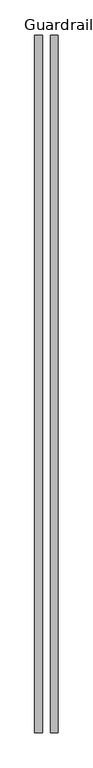
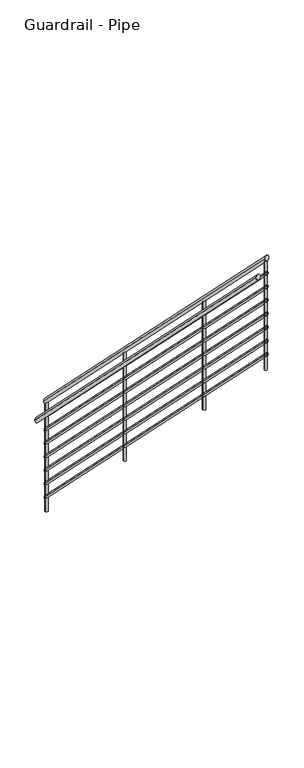
"""IFC4 building model written with IfcOpenShell, lengths in millimetres: railing geometry, Guardrail - Pipe."""

import ifcopenshell
import ifcopenshell.guid

model = None  # the IFC model being written
_history = None  # IfcOwnerHistory: only IFC2X3 demands one
_inside = {}  # id of a spatial element -> (the spatial element, [elements in it])
_under = {}  # id of a project, library or spatial element -> (it, [spatial elements below it])
_declared = {}  # id of a project -> (the project, [libraries it declares])
_typed = {}  # id of a type object -> (the type object, [elements of that type])
_made_of = {}  # id of a material, layer set ... -> (it, [elements and type objects made of it])


def new_model(schema):
    """Start an empty IFC model of exactly this schema.

    Asked for "IFC4X3", IfcOpenShell would pick the latest addendum, in which some entities
    have other attributes; the version numbers below select the first issue.
    IFC2X3 requires an IfcOwnerHistory on every rooted entity: one is made here for all.
    """
    global model, _history
    if schema == "IFC4X3":
        model = ifcopenshell.file(schema_version=(4, 3, 0, 0))
    else:
        model = ifcopenshell.file(schema=schema)
    _inside.clear()
    _under.clear()
    _declared.clear()
    _typed.clear()
    _made_of.clear()
    _history = None
    if model.schema == "IFC2X3":
        org = make("IfcOrganization", Name="unknown")
        user = make(
            "IfcPersonAndOrganization",
            ThePerson=make("IfcPerson", FamilyName="unknown"),
            TheOrganization=org,
        )
        app = make(
            "IfcApplication",
            ApplicationDeveloper=org,
            Version="unknown",
            ApplicationFullName="unknown",
            ApplicationIdentifier="unknown",
        )
        _history = make(
            "IfcOwnerHistory",
            OwningUser=user,
            OwningApplication=app,
            ChangeAction="ADDED",
            CreationDate=0,
        )
    return model


def make(cls, **values):
    """One entity of the class cls with the attributes given. An attribute that is None is left unset."""
    return model.create_entity(
        cls, **{name: value for name, value in values.items() if value is not None}
    )


def rooted(cls, **values):
    """An entity with a GlobalId (a new one), such as an element, a storey or a relation."""
    return make(cls, GlobalId=ifcopenshell.guid.new(), OwnerHistory=_history, **values)


def si_unit(unit_type, name, prefix=None):
    """IfcSIUnit, for example si_unit("LENGTHUNIT", "METRE", prefix="MILLI")."""
    return make("IfcSIUnit", UnitType=unit_type, Prefix=prefix, Name=name)


def assignment(units):
    """IfcUnitAssignment: the units of a project."""
    return None if units is None else make("IfcUnitAssignment", Units=units)


def point(xyz):
    """IfcCartesianPoint."""
    return None if xyz is None else make("IfcCartesianPoint", Coordinates=xyz)


def direction(xyz):
    """IfcDirection."""
    return None if xyz is None else make("IfcDirection", DirectionRatios=xyz)


def frame(location, z_axis=None, x_axis=None):
    """IfcAxis2Placement3D, a coordinate frame: its origin and axes. An axis left out is left unset."""
    return make(
        "IfcAxis2Placement3D",
        Location=point(location),
        Axis=direction(z_axis),
        RefDirection=direction(x_axis),
    )


def origin():
    """The frame at (0, 0, 0) with its axes left unset."""
    return frame((0.0, 0.0, 0.0))


def place(relative_to, where):
    """IfcLocalPlacement: puts the frame where relative to a parent placement (None: the world)."""
    return make(
        "IfcLocalPlacement", PlacementRelTo=relative_to, RelativePlacement=where
    )


def context(
    kind, dimensions, precision=None, world=None, true_north=None, identifier=None
):
    """IfcGeometricRepresentationContext, for example the 3D "Model" context."""
    return make(
        "IfcGeometricRepresentationContext",
        ContextIdentifier=identifier,
        ContextType=kind,
        CoordinateSpaceDimension=dimensions,
        Precision=precision,
        WorldCoordinateSystem=world,
        TrueNorth=true_north,
    )


def project(units=None, contexts=None):
    """IfcProject with its units and contexts."""
    return rooted(
        "IfcProject",
        Name="project",
        RepresentationContexts=contexts,
        UnitsInContext=assignment(units),
    )


def spatial(cls, under=None, at=None, **own):
    """A site, building, storey or space (cls), placed at a placement, below another one or the project."""
    s = rooted(cls, ObjectPlacement=at, **own)
    if under is not None:
        _under.setdefault(under.id(), (under, []))[1].append(s)
    return s


def circle_curve(where, radius):
    """IfcCircle in the frame where."""
    return make("IfcCircle", Position=where, Radius=radius)


def ellipse_curve(where, semi_axis1, semi_axis2):
    """IfcEllipse in the frame where."""
    return make(
        "IfcEllipse", Position=where, SemiAxis1=semi_axis1, SemiAxis2=semi_axis2
    )


def shape(context_of_items, identifier, shape_type, items):
    """IfcShapeRepresentation: the items that make up one representation, for example the "Body"."""
    return make(
        "IfcShapeRepresentation",
        ContextOfItems=context_of_items,
        RepresentationIdentifier=identifier,
        RepresentationType=shape_type,
        Items=items,
    )


def source(mapping_origin, context_of_items, identifier, shape_type, items):
    """IfcRepresentationMap: a shape defined once, which mapped items show again and again."""
    return make(
        "IfcRepresentationMap",
        MappingOrigin=mapping_origin,
        MappedRepresentation=shape(context_of_items, identifier, shape_type, items),
    )


def transform(
    local_origin,
    x_axis=None,
    y_axis=None,
    z_axis=None,
    scale=None,
    scale2=None,
    scale3=None,
    uniform=True,
):
    """IfcCartesianTransformationOperator3D, or its non-uniform kind. x_axis, y_axis, z_axis: its Axis1, 2, 3."""
    if uniform:
        return make(
            "IfcCartesianTransformationOperator3D",
            Axis1=direction(x_axis),
            Axis2=direction(y_axis),
            LocalOrigin=point(local_origin),
            Scale=scale,
            Axis3=direction(z_axis),
        )
    return make(
        "IfcCartesianTransformationOperator3DnonUniform",
        Axis1=direction(x_axis),
        Axis2=direction(y_axis),
        LocalOrigin=point(local_origin),
        Scale=scale,
        Axis3=direction(z_axis),
        Scale2=scale2,
        Scale3=scale3,
    )


def mapped(mapping_source, mapping_target):
    """IfcMappedItem: shows the shape of a source again, moved by a transform."""
    return make(
        "IfcMappedItem", MappingSource=mapping_source, MappingTarget=mapping_target
    )


def made_of(thing, what):
    """Note that an element or type object is made of a material, layer set ...; save() writes the relation."""
    if what is not None:
        _made_of.setdefault(what.id(), (what, []))[1].append(thing)
    return thing


def element(
    cls,
    number,
    at=None,
    inside=None,
    cuts=None,
    type_object=None,
    material=None,
    context=None,
    identifier="Body",
    shape_type=None,
    held_by="IfcProductDefinitionShape",
    body=None,
    shapes=None,
    **own,
):
    """One element of the class cls, such as IfcWall. Its Tag is "e" and its number.

    at: its placement. inside: the storey or other place that contains it. cuts: it is an
    opening in that element (IfcRelVoidsElement). A single representation is given by context,
    identifier, shape_type and body (its items); several are given by shapes. held_by: the class
    of the entity that holds the representations. save() writes the other relations.
    """
    e = rooted(cls, Tag="e%d" % number, ObjectPlacement=at, **own)
    if body is not None:
        shapes = [shape(context, identifier, shape_type, body)]
    if shapes is not None:
        e.Representation = make(held_by, Representations=shapes)
    if inside is not None:
        _inside.setdefault(inside.id(), (inside, []))[1].append(e)
    if cuts is not None:
        rooted(
            "IfcRelVoidsElement", RelatingBuildingElement=cuts, RelatedOpeningElement=e
        )
    if type_object is not None:
        _typed.setdefault(type_object.id(), (type_object, []))[1].append(e)
    return made_of(e, material)


def aggregate(whole, parts):
    """IfcRelAggregates: a whole, such as a stair, and the parts it consists of."""
    return rooted("IfcRelAggregates", RelatingObject=whole, RelatedObjects=parts)


def save(model, path):
    """Write the relations noted so far, then the file.

    IfcRelAggregates (storeys below a building ...), IfcRelContainedInSpatialStructure (elements
    in a storey), IfcRelDefinesByType, IfcRelAssociatesMaterial and IfcRelDeclares: one each for
    every whole, place, type object, material and project.
    """
    for whole, parts in _under.values():
        aggregate(whole, parts)
    for where, things in _inside.values():
        rooted(
            "IfcRelContainedInSpatialStructure",
            RelatedElements=things,
            RelatingStructure=where,
        )
    for kind, things in _typed.values():
        rooted("IfcRelDefinesByType", RelatedObjects=things, RelatingType=kind)
    for what, things in _made_of.values():
        rooted("IfcRelAssociatesMaterial", RelatedObjects=things, RelatingMaterial=what)
    for by, libraries in _declared.values():
        rooted("IfcRelDeclares", RelatingContext=by, RelatedDefinitions=libraries)
    model.write(path)


def plane_surface(at):
    """IfcPlane: the flat surface through the origin of the frame at, square to its z axis."""
    return make("IfcPlane", Position=at)


def cylinder_surface(at, radius):
    """IfcCylindricalSurface: all points at the distance radius from the z axis of the frame at."""
    return make("IfcCylindricalSurface", Position=at, Radius=radius)


def advanced_brep(points, edges, surfaces, faces):
    """IfcAdvancedBrep: a solid bounded by faces that lie on surfaces and meet in shared edges.

    An edge is (start, end): straight between two places in points (the first is 0);
    or (start, end, curve); or (start, end, curve, False) where it runs against its curve.
    A face is (place in surfaces, loops), or (place, loops, False) where it looks against
    its surface's normal. A loop lists edges by number (the first is 1), with a minus sign
    where the edge is run from its end to its start. The first loop is the outer one.
    """
    corners = [point(p) for p in points]
    vertices = [make("IfcVertexPoint", VertexGeometry=c) for c in corners]
    made = []
    for start, end, *more in edges:
        made.append(
            make(
                "IfcEdgeCurve",
                EdgeStart=vertices[start],
                EdgeEnd=vertices[end],
                EdgeGeometry=more[0] if more else make("IfcPolyline", Points=[corners[start], corners[end]]),
                SameSense=more[1] if len(more) > 1 else True,
            )
        )
    hull = []
    for where, loops, *sense in faces:
        bounds = []
        for j, loop in enumerate(loops):
            ring = [make("IfcOrientedEdge", EdgeElement=made[abs(k) - 1], Orientation=k > 0) for k in loop]
            bounds.append(
                make(
                    "IfcFaceOuterBound" if j == 0 else "IfcFaceBound",
                    Bound=make("IfcEdgeLoop", EdgeList=ring),
                    Orientation=True,
                )
            )
        hull.append(make("IfcAdvancedFace", Bounds=bounds, FaceSurface=surfaces[where], SameSense=sense[0] if sense else True))
    return make("IfcAdvancedBrep", Outer=make("IfcClosedShell", CfsFaces=hull))


def guardrail_pipe_ffde7d2e(model_context):
    return source(origin(), model_context, "Body", "AdvancedBrep", [
        advanced_brep(
        [(-590.6362718, 32344.1921646, 1268.4592316), (-552.5362718, 32344.1921646, 1268.4592316), (-590.6362718, 28942.3977925, 4670.2536037), (-552.5362718, 28942.3977925, 4670.2536037)],
        [
            (0, 1, ellipse_curve(frame((-571.5862718, 32344.1921646, 1268.4592316), z_axis=(0.0, 1.0, 0.0), x_axis=(0.0, 0.0, -1.0)), 26.9407684, 19.05)),
            (1, 0, ellipse_curve(frame((-571.5862718, 32344.1921646, 1268.4592316), z_axis=(0.0, 1.0, 0.0), x_axis=(0.0, 0.0, -1.0)), 26.9407684, 19.05)),
            (2, 3, ellipse_curve(frame((-571.5862718, 28942.3977925, 4670.2536037), z_axis=(0.0, -1.0, 0.0), x_axis=(0.0, 0.0, -1.0)), 26.9407684, 19.05)),
            (3, 2, ellipse_curve(frame((-571.5862718, 28942.3977925, 4670.2536037), z_axis=(0.0, -1.0, 0.0), x_axis=(0.0, 0.0, -1.0)), 26.9407684, 19.05)),
            (0, 2),
            (3, 1),
        ],
        [
            plane_surface(frame((-571.5862718, 32344.1921646, 1295.4), z_axis=(0.0, 1.0, 0.0), x_axis=(0.0, 0.0, -1.0))),
            plane_surface(frame((-571.5862718, 28942.3977925, 4697.194372), z_axis=(0.0, -1.0, 0.0), x_axis=(0.0, 0.0, -1.0))),
            cylinder_surface(frame((-571.5862718, 32330.7217804, 1281.9296158), z_axis=(0.0, 0.7071067811865476, -0.7071067811865476), x_axis=(1.0, 0.0, 0.0)), 19.05),
        ],
        [
            (0, [[1, 2]]),
            (1, [[3, 4]]),
            (2, [[-1, 5, -4, 6]]),
            (2, [[-2, -6, -3, -5]]),
        ],
    ),
        advanced_brep(
        [(-584.2862718, 32344.1921646, 1125.0394878), (-558.8862718, 32344.1921646, 1125.0394878), (-584.2862718, 28942.3977925, 4526.8338598), (-558.8862718, 28942.3977925, 4526.8338598)],
        [
            (0, 1, ellipse_curve(frame((-571.5862718, 32344.1921646, 1125.0394878), z_axis=(0.0, 1.0, 0.0), x_axis=(0.0, 0.0, -1.0)), 17.9605122, 12.7)),
            (1, 0, ellipse_curve(frame((-571.5862718, 32344.1921646, 1125.0394878), z_axis=(0.0, 1.0, 0.0), x_axis=(0.0, 0.0, -1.0)), 17.9605122, 12.7)),
            (2, 3, ellipse_curve(frame((-571.5862718, 28942.3977925, 4526.8338598), z_axis=(0.0, -1.0, 0.0), x_axis=(0.0, 0.0, -1.0)), 17.9605122, 12.7)),
            (3, 2, ellipse_curve(frame((-571.5862718, 28942.3977925, 4526.8338598), z_axis=(0.0, -1.0, 0.0), x_axis=(0.0, 0.0, -1.0)), 17.9605122, 12.7)),
            (0, 2),
            (3, 1),
        ],
        [
            plane_surface(frame((-571.5862718, 32344.1921646, 1143.0), z_axis=(0.0, 1.0, 0.0), x_axis=(0.0, 0.0, -1.0))),
            plane_surface(frame((-571.5862718, 28942.3977925, 4544.794372), z_axis=(0.0, -1.0, 0.0), x_axis=(0.0, 0.0, -1.0))),
            cylinder_surface(frame((-571.5862718, 32335.2119084, 1134.0197439), z_axis=(0.0, 0.7071067811865476, -0.7071067811865476), x_axis=(1.0, 0.0, 0.0)), 12.7),
        ],
        [
            (0, [[1, 2]]),
            (1, [[3, 4]]),
            (2, [[-1, 5, -4, 6]]),
            (2, [[-2, -6, -3, -5]]),
        ],
    ),
        advanced_brep(
        [(-666.8362718, 32344.1921646, 1116.0592316), (-628.7362718, 32344.1921646, 1116.0592316), (-666.8362718, 28942.3977925, 4517.8536037), (-628.7362718, 28942.3977925, 4517.8536037)],
        [
            (0, 1, ellipse_curve(frame((-647.7862718, 32344.1921646, 1116.0592316), z_axis=(0.0, 1.0, 0.0), x_axis=(0.0, 0.0, -1.0)), 26.9407684, 19.05)),
            (1, 0, ellipse_curve(frame((-647.7862718, 32344.1921646, 1116.0592316), z_axis=(0.0, 1.0, 0.0), x_axis=(0.0, 0.0, -1.0)), 26.9407684, 19.05)),
            (2, 3, ellipse_curve(frame((-647.7862718, 28942.3977925, 4517.8536037), z_axis=(0.0, -1.0, 0.0), x_axis=(0.0, 0.0, -1.0)), 26.9407684, 19.05)),
            (3, 2, ellipse_curve(frame((-647.7862718, 28942.3977925, 4517.8536037), z_axis=(0.0, -1.0, 0.0), x_axis=(0.0, 0.0, -1.0)), 26.9407684, 19.05)),
            (0, 2),
            (3, 1),
        ],
        [
            plane_surface(frame((-647.7862718, 32344.1921646, 1143.0), z_axis=(0.0, 1.0, 0.0), x_axis=(0.0, 0.0, -1.0))),
            plane_surface(frame((-647.7862718, 28942.3977925, 4544.794372), z_axis=(0.0, -1.0, 0.0), x_axis=(0.0, 0.0, -1.0))),
            cylinder_surface(frame((-647.7862718, 32330.7217804, 1129.5296158), z_axis=(0.0, 0.7071067811865476, -0.7071067811865476), x_axis=(1.0, 0.0, 0.0)), 19.05),
        ],
        [
            (0, [[1, 2]]),
            (1, [[3, 4]]),
            (2, [[-1, 5, -4, 6]]),
            (2, [[-2, -6, -3, -5]]),
        ],
    ),
        advanced_brep(
        [(-584.2862718, 32344.1921646, 998.0394878), (-558.8862718, 32344.1921646, 998.0394878), (-584.2862718, 28942.3977925, 4399.8338598), (-558.8862718, 28942.3977925, 4399.8338598)],
        [
            (0, 1, ellipse_curve(frame((-571.5862718, 32344.1921646, 998.0394878), z_axis=(0.0, 1.0, 0.0), x_axis=(0.0, 0.0, -1.0)), 17.9605122, 12.7)),
            (1, 0, ellipse_curve(frame((-571.5862718, 32344.1921646, 998.0394878), z_axis=(0.0, 1.0, 0.0), x_axis=(0.0, 0.0, -1.0)), 17.9605122, 12.7)),
            (2, 3, ellipse_curve(frame((-571.5862718, 28942.3977925, 4399.8338598), z_axis=(0.0, -1.0, 0.0), x_axis=(0.0, 0.0, -1.0)), 17.9605122, 12.7)),
            (3, 2, ellipse_curve(frame((-571.5862718, 28942.3977925, 4399.8338598), z_axis=(0.0, -1.0, 0.0), x_axis=(0.0, 0.0, -1.0)), 17.9605122, 12.7)),
            (0, 2),
            (3, 1),
        ],
        [
            plane_surface(frame((-571.5862718, 32344.1921646, 1016.0), z_axis=(0.0, 1.0, 0.0), x_axis=(0.0, 0.0, -1.0))),
            plane_surface(frame((-571.5862718, 28942.3977925, 4417.794372), z_axis=(0.0, -1.0, 0.0), x_axis=(0.0, 0.0, -1.0))),
            cylinder_surface(frame((-571.5862718, 32335.2119084, 1007.0197439), z_axis=(0.0, 0.7071067811865476, -0.7071067811865476), x_axis=(1.0, 0.0, 0.0)), 12.7),
        ],
        [
            (0, [[1, 2]]),
            (1, [[3, 4]]),
            (2, [[-1, 5, -4, 6]]),
            (2, [[-2, -6, -3, -5]]),
        ],
    ),
        advanced_brep(
        [(-584.2862718, 32344.1921646, 871.0394878), (-558.8862718, 32344.1921646, 871.0394878), (-584.2862718, 28942.3977925, 4272.8338598), (-558.8862718, 28942.3977925, 4272.8338598)],
        [
            (0, 1, ellipse_curve(frame((-571.5862718, 32344.1921646, 871.0394878), z_axis=(0.0, 1.0, 0.0), x_axis=(0.0, 0.0, -1.0)), 17.9605122, 12.7)),
            (1, 0, ellipse_curve(frame((-571.5862718, 32344.1921646, 871.0394878), z_axis=(0.0, 1.0, 0.0), x_axis=(0.0, 0.0, -1.0)), 17.9605122, 12.7)),
            (2, 3, ellipse_curve(frame((-571.5862718, 28942.3977925, 4272.8338598), z_axis=(0.0, -1.0, 0.0), x_axis=(0.0, 0.0, -1.0)), 17.9605122, 12.7)),
            (3, 2, ellipse_curve(frame((-571.5862718, 28942.3977925, 4272.8338598), z_axis=(0.0, -1.0, 0.0), x_axis=(0.0, 0.0, -1.0)), 17.9605122, 12.7)),
            (0, 2),
            (3, 1),
        ],
        [
            plane_surface(frame((-571.5862718, 32344.1921646, 889.0), z_axis=(0.0, 1.0, 0.0), x_axis=(0.0, 0.0, -1.0))),
            plane_surface(frame((-571.5862718, 28942.3977925, 4290.794372), z_axis=(0.0, -1.0, 0.0), x_axis=(0.0, 0.0, -1.0))),
            cylinder_surface(frame((-571.5862718, 32335.2119084, 880.0197439), z_axis=(0.0, 0.7071067811865476, -0.7071067811865476), x_axis=(1.0, 0.0, 0.0)), 12.7),
        ],
        [
            (0, [[1, 2]]),
            (1, [[3, 4]]),
            (2, [[-1, 5, -4, 6]]),
            (2, [[-2, -6, -3, -5]]),
        ],
    ),
        advanced_brep(
        [(-584.2862718, 32344.1921646, 744.0394878), (-558.8862718, 32344.1921646, 744.0394878), (-584.2862718, 28942.3977925, 4145.8338598), (-558.8862718, 28942.3977925, 4145.8338598)],
        [
            (0, 1, ellipse_curve(frame((-571.5862718, 32344.1921646, 744.0394878), z_axis=(0.0, 1.0, 0.0), x_axis=(0.0, 0.0, -1.0)), 17.9605122, 12.7)),
            (1, 0, ellipse_curve(frame((-571.5862718, 32344.1921646, 744.0394878), z_axis=(0.0, 1.0, 0.0), x_axis=(0.0, 0.0, -1.0)), 17.9605122, 12.7)),
            (2, 3, ellipse_curve(frame((-571.5862718, 28942.3977925, 4145.8338598), z_axis=(0.0, -1.0, 0.0), x_axis=(0.0, 0.0, -1.0)), 17.9605122, 12.7)),
            (3, 2, ellipse_curve(frame((-571.5862718, 28942.3977925, 4145.8338598), z_axis=(0.0, -1.0, 0.0), x_axis=(0.0, 0.0, -1.0)), 17.9605122, 12.7)),
            (0, 2),
            (3, 1),
        ],
        [
            plane_surface(frame((-571.5862718, 32344.1921646, 762.0), z_axis=(0.0, 1.0, 0.0), x_axis=(0.0, 0.0, -1.0))),
            plane_surface(frame((-571.5862718, 28942.3977925, 4163.794372), z_axis=(0.0, -1.0, 0.0), x_axis=(0.0, 0.0, -1.0))),
            cylinder_surface(frame((-571.5862718, 32335.2119084, 753.0197439), z_axis=(0.0, 0.7071067811865476, -0.7071067811865476), x_axis=(1.0, 0.0, 0.0)), 12.7),
        ],
        [
            (0, [[1, 2]]),
            (1, [[3, 4]]),
            (2, [[-1, 5, -4, 6]]),
            (2, [[-2, -6, -3, -5]]),
        ],
    ),
        advanced_brep(
        [(-584.2862718, 32344.1921646, 617.0394878), (-558.8862718, 32344.1921646, 617.0394878), (-584.2862718, 28942.3977925, 4018.8338598), (-558.8862718, 28942.3977925, 4018.8338598)],
        [
            (0, 1, ellipse_curve(frame((-571.5862718, 32344.1921646, 617.0394878), z_axis=(0.0, 1.0, 0.0), x_axis=(0.0, 0.0, -1.0)), 17.9605122, 12.7)),
            (1, 0, ellipse_curve(frame((-571.5862718, 32344.1921646, 617.0394878), z_axis=(0.0, 1.0, 0.0), x_axis=(0.0, 0.0, -1.0)), 17.9605122, 12.7)),
            (2, 3, ellipse_curve(frame((-571.5862718, 28942.3977925, 4018.8338598), z_axis=(0.0, -1.0, 0.0), x_axis=(0.0, 0.0, -1.0)), 17.9605122, 12.7)),
            (3, 2, ellipse_curve(frame((-571.5862718, 28942.3977925, 4018.8338598), z_axis=(0.0, -1.0, 0.0), x_axis=(0.0, 0.0, -1.0)), 17.9605122, 12.7)),
            (0, 2),
            (3, 1),
        ],
        [
            plane_surface(frame((-571.5862718, 32344.1921646, 635.0), z_axis=(0.0, 1.0, 0.0), x_axis=(0.0, 0.0, -1.0))),
            plane_surface(frame((-571.5862718, 28942.3977925, 4036.794372), z_axis=(0.0, -1.0, 0.0), x_axis=(0.0, 0.0, -1.0))),
            cylinder_surface(frame((-571.5862718, 32335.2119084, 626.0197439), z_axis=(0.0, 0.7071067811865476, -0.7071067811865476), x_axis=(1.0, 0.0, 0.0)), 12.7),
        ],
        [
            (0, [[1, 2]]),
            (1, [[3, 4]]),
            (2, [[-1, 5, -4, 6]]),
            (2, [[-2, -6, -3, -5]]),
        ],
    ),
        advanced_brep(
        [(-584.2862718, 32344.1921646, 490.0394878), (-558.8862718, 32344.1921646, 490.0394878), (-584.2862718, 28942.3977925, 3891.8338598), (-558.8862718, 28942.3977925, 3891.8338598)],
        [
            (0, 1, ellipse_curve(frame((-571.5862718, 32344.1921646, 490.0394878), z_axis=(0.0, 1.0, 0.0), x_axis=(0.0, 0.0, -1.0)), 17.9605122, 12.7)),
            (1, 0, ellipse_curve(frame((-571.5862718, 32344.1921646, 490.0394878), z_axis=(0.0, 1.0, 0.0), x_axis=(0.0, 0.0, -1.0)), 17.9605122, 12.7)),
            (2, 3, ellipse_curve(frame((-571.5862718, 28942.3977925, 3891.8338598), z_axis=(0.0, -1.0, 0.0), x_axis=(0.0, 0.0, -1.0)), 17.9605122, 12.7)),
            (3, 2, ellipse_curve(frame((-571.5862718, 28942.3977925, 3891.8338598), z_axis=(0.0, -1.0, 0.0), x_axis=(0.0, 0.0, -1.0)), 17.9605122, 12.7)),
            (0, 2),
            (3, 1),
        ],
        [
            plane_surface(frame((-571.5862718, 32344.1921646, 508.0), z_axis=(0.0, 1.0, 0.0), x_axis=(0.0, 0.0, -1.0))),
            plane_surface(frame((-571.5862718, 28942.3977925, 3909.794372), z_axis=(0.0, -1.0, 0.0), x_axis=(0.0, 0.0, -1.0))),
            cylinder_surface(frame((-571.5862718, 32335.2119084, 499.0197439), z_axis=(0.0, 0.7071067811865476, -0.7071067811865476), x_axis=(1.0, 0.0, 0.0)), 12.7),
        ],
        [
            (0, [[1, 2]]),
            (1, [[3, 4]]),
            (2, [[-1, 5, -4, 6]]),
            (2, [[-2, -6, -3, -5]]),
        ],
    ),
        advanced_brep(
        [(-584.2862718, 32344.1921646, 363.0394878), (-558.8862718, 32344.1921646, 363.0394878), (-584.2862718, 28942.3977925, 3764.8338598), (-558.8862718, 28942.3977925, 3764.8338598)],
        [
            (0, 1, ellipse_curve(frame((-571.5862718, 32344.1921646, 363.0394878), z_axis=(0.0, 1.0, 0.0), x_axis=(0.0, 0.0, -1.0)), 17.9605122, 12.7)),
            (1, 0, ellipse_curve(frame((-571.5862718, 32344.1921646, 363.0394878), z_axis=(0.0, 1.0, 0.0), x_axis=(0.0, 0.0, -1.0)), 17.9605122, 12.7)),
            (2, 3, ellipse_curve(frame((-571.5862718, 28942.3977925, 3764.8338598), z_axis=(0.0, -1.0, 0.0), x_axis=(0.0, 0.0, -1.0)), 17.9605122, 12.7)),
            (3, 2, ellipse_curve(frame((-571.5862718, 28942.3977925, 3764.8338598), z_axis=(0.0, -1.0, 0.0), x_axis=(0.0, 0.0, -1.0)), 17.9605122, 12.7)),
            (0, 2),
            (3, 1),
        ],
        [
            plane_surface(frame((-571.5862718, 32344.1921646, 381.0), z_axis=(0.0, 1.0, 0.0), x_axis=(0.0, 0.0, -1.0))),
            plane_surface(frame((-571.5862718, 28942.3977925, 3782.794372), z_axis=(0.0, -1.0, 0.0), x_axis=(0.0, 0.0, -1.0))),
            cylinder_surface(frame((-571.5862718, 32335.2119084, 372.0197439), z_axis=(0.0, 0.7071067811865476, -0.7071067811865476), x_axis=(1.0, 0.0, 0.0)), 12.7),
        ],
        [
            (0, [[1, 2]]),
            (1, [[3, 4]]),
            (2, [[-1, 5, -4, 6]]),
            (2, [[-2, -6, -3, -5]]),
        ],
    ),
        advanced_brep(
        [(-558.8862718, 29905.7921646, 3679.9184633), (-584.2862718, 29905.7921646, 3679.9184633), (-584.2862718, 29905.7921646, 2667.0), (-558.8862718, 29905.7921646, 2667.0)],
        [
            (0, 1, ellipse_curve(frame((-571.5862718, 29905.7921646, 3679.9184633), z_axis=(0.0, -0.7071067811865471, -0.7071067811865479), x_axis=(0.0, -0.7071067811865479, 0.7071067811865471)), 17.9605122, 12.7)),
            (1, 2),
            (2, 3, circle_curve(frame((-571.5862718, 29905.7921646, 2667.0), z_axis=(0.0, 0.0, 1.0), x_axis=(-1.0, 0.0, 0.0)), 12.7)),
            (3, 0),
            (3, 2, circle_curve(frame((-571.5862718, 29905.7921646, 2667.0), z_axis=(0.0, 0.0, 1.0), x_axis=(-1.0, 0.0, 0.0)), 12.7)),
            (1, 0, ellipse_curve(frame((-571.5862718, 29905.7921646, 3679.9184633), z_axis=(0.0, -0.7071067811865471, -0.7071067811865479), x_axis=(0.0, -0.7071067811865479, 0.7071067811865471)), 17.9605122, 12.7)),
        ],
        [
            cylinder_surface(frame((-571.5862718, 29905.7921646, 2438.4), z_axis=(0.0, 0.0, 1.0), x_axis=(-1.0, 0.0, 0.0)), 12.7),
            plane_surface(frame((-596.9862718, 29880.3921646, 3705.3184633), z_axis=(0.0, 0.7071067811865471, 0.7071067811865479), x_axis=(1.0, 0.0, 0.0))),
            plane_surface(frame((-596.9862718, 29931.1921646, 2667.0), z_axis=(0.0, 0.0, -1.0), x_axis=(1.0, 0.0, 0.0))),
        ],
        [
            (0, [[1, 2, 3, 4]]),
            (0, [[5, -2, 6, -4]]),
            (1, [[-6, -1]]),
            (2, [[-5, -3]]),
        ],
    ),
        advanced_brep(
        [(-558.8862718, 31124.9921646, 2460.7184633), (-584.2862718, 31124.9921646, 2460.7184633), (-584.2862718, 31124.9921646, 1447.8), (-558.8862718, 31124.9921646, 1447.8)],
        [
            (0, 1, ellipse_curve(frame((-571.5862718, 31124.9921646, 2460.7184633), z_axis=(0.0, -0.7071067811865471, -0.7071067811865479), x_axis=(0.0, -0.7071067811865479, 0.7071067811865471)), 17.9605122, 12.7)),
            (1, 2),
            (2, 3, circle_curve(frame((-571.5862718, 31124.9921646, 1447.8), z_axis=(0.0, 0.0, 1.0), x_axis=(-1.0, 0.0, 0.0)), 12.7)),
            (3, 0),
            (3, 2, circle_curve(frame((-571.5862718, 31124.9921646, 1447.8), z_axis=(0.0, 0.0, 1.0), x_axis=(-1.0, 0.0, 0.0)), 12.7)),
            (1, 0, ellipse_curve(frame((-571.5862718, 31124.9921646, 2460.7184633), z_axis=(0.0, -0.7071067811865471, -0.7071067811865479), x_axis=(0.0, -0.7071067811865479, 0.7071067811865471)), 17.9605122, 12.7)),
        ],
        [
            cylinder_surface(frame((-571.5862718, 31124.9921646, 1219.2), z_axis=(0.0, 0.0, 1.0), x_axis=(-1.0, 0.0, 0.0)), 12.7),
            plane_surface(frame((-596.9862718, 31099.5921646, 2486.1184633), z_axis=(0.0, 0.7071067811865471, 0.7071067811865479), x_axis=(1.0, 0.0, 0.0))),
            plane_surface(frame((-596.9862718, 31150.3921646, 1447.8), z_axis=(0.0, 0.0, -1.0), x_axis=(1.0, 0.0, 0.0))),
        ],
        [
            (0, [[1, 2, 3, 4]]),
            (0, [[5, -2, 6, -4]]),
            (1, [[-6, -1]]),
            (2, [[-5, -3]]),
        ],
    ),
        advanced_brep(
        [(-558.8862718, 28955.0977925, 4630.6128353), (-584.2862718, 28955.0977925, 4630.6128353), (-584.2862718, 28955.0977925, 3617.694372), (-558.8862718, 28955.0977925, 3617.694372)],
        [
            (0, 1, ellipse_curve(frame((-571.5862718, 28955.0977925, 4630.6128353), z_axis=(0.0, -0.7071067811865471, -0.7071067811865479), x_axis=(0.0, -0.7071067811865479, 0.7071067811865471)), 17.9605122, 12.7)),
            (1, 2),
            (2, 3, circle_curve(frame((-571.5862718, 28955.0977925, 3617.694372), z_axis=(0.0, 0.0, 1.0), x_axis=(-1.0, 0.0, 0.0)), 12.7)),
            (3, 0),
            (3, 2, circle_curve(frame((-571.5862718, 28955.0977925, 3617.694372), z_axis=(0.0, 0.0, 1.0), x_axis=(-1.0, 0.0, 0.0)), 12.7)),
            (1, 0, ellipse_curve(frame((-571.5862718, 28955.0977925, 4630.6128353), z_axis=(0.0, -0.7071067811865471, -0.7071067811865479), x_axis=(0.0, -0.7071067811865479, 0.7071067811865471)), 17.9605122, 12.7)),
        ],
        [
            cylinder_surface(frame((-571.5862718, 28955.0977925, 3389.094372), z_axis=(0.0, 0.0, 1.0), x_axis=(-1.0, 0.0, 0.0)), 12.7),
            plane_surface(frame((-596.9862718, 28929.6977925, 4656.0128353), z_axis=(0.0, 0.7071067811865471, 0.7071067811865479), x_axis=(1.0, 0.0, 0.0))),
            plane_surface(frame((-596.9862718, 28980.4977925, 3617.694372), z_axis=(0.0, 0.0, -1.0), x_axis=(1.0, 0.0, 0.0))),
        ],
        [
            (0, [[1, 2, 3, 4]]),
            (0, [[5, -2, 6, -4]]),
            (1, [[-6, -1]]),
            (2, [[-5, -3]]),
        ],
    ),
        advanced_brep(
        [(-558.8862718, 32331.4921646, 1254.2184633), (-584.2862718, 32331.4921646, 1254.2184633), (-584.2862718, 32331.4921646, 241.3), (-558.8862718, 32331.4921646, 241.3)],
        [
            (0, 1, ellipse_curve(frame((-571.5862718, 32331.4921646, 1254.2184633), z_axis=(0.0, -0.7071067811865471, -0.7071067811865479), x_axis=(0.0, -0.7071067811865479, 0.7071067811865471)), 17.9605122, 12.7)),
            (1, 2),
            (2, 3, circle_curve(frame((-571.5862718, 32331.4921646, 241.3), z_axis=(0.0, 0.0, 1.0), x_axis=(-1.0, 0.0, 0.0)), 12.7)),
            (3, 0),
            (3, 2, circle_curve(frame((-571.5862718, 32331.4921646, 241.3), z_axis=(0.0, 0.0, 1.0), x_axis=(-1.0, 0.0, 0.0)), 12.7)),
            (1, 0, ellipse_curve(frame((-571.5862718, 32331.4921646, 1254.2184633), z_axis=(0.0, -0.7071067811865471, -0.7071067811865479), x_axis=(0.0, -0.7071067811865479, 0.7071067811865471)), 17.9605122, 12.7)),
        ],
        [
            cylinder_surface(frame((-571.5862718, 32331.4921646, 12.7), z_axis=(0.0, 0.0, 1.0), x_axis=(-1.0, 0.0, 0.0)), 12.7),
            plane_surface(frame((-596.9862718, 32306.0921646, 1279.6184633), z_axis=(0.0, 0.7071067811865471, 0.7071067811865479), x_axis=(1.0, 0.0, 0.0))),
            plane_surface(frame((-596.9862718, 32356.8921646, 241.3), z_axis=(0.0, 0.0, -1.0), x_axis=(1.0, 0.0, 0.0))),
        ],
        [
            (0, [[1, 2, 3, 4]]),
            (0, [[5, -2, 6, -4]]),
            (1, [[-6, -1]]),
            (2, [[-5, -3]]),
        ],
    ),
    ])


if __name__ == "__main__":
    model = new_model("IFC4")
    model_context = context("Model", 3, world=origin())
    ifc_project = project(units=[si_unit("LENGTHUNIT", "METRE", prefix="MILLI")], contexts=[model_context])
    site = spatial("IfcSite", under=ifc_project)
    building = spatial("IfcBuilding", under=site)
    placement = place(None, origin())
    guardrail_pipe_shape = guardrail_pipe_ffde7d2e(model_context)
    element("IfcRailing", 1, ObjectType="Guardrail - Pipe", at=placement, inside=building, context=model_context, shape_type="MappedRepresentation", body=[
        mapped(guardrail_pipe_shape, transform((0.0, 0.0, 0.0), x_axis=(1.0, 0.0, 0.0), y_axis=(0.0, 1.0, 0.0), z_axis=(0.0, 0.0, 1.0))),
    ])
    save(model, "model.ifc")
